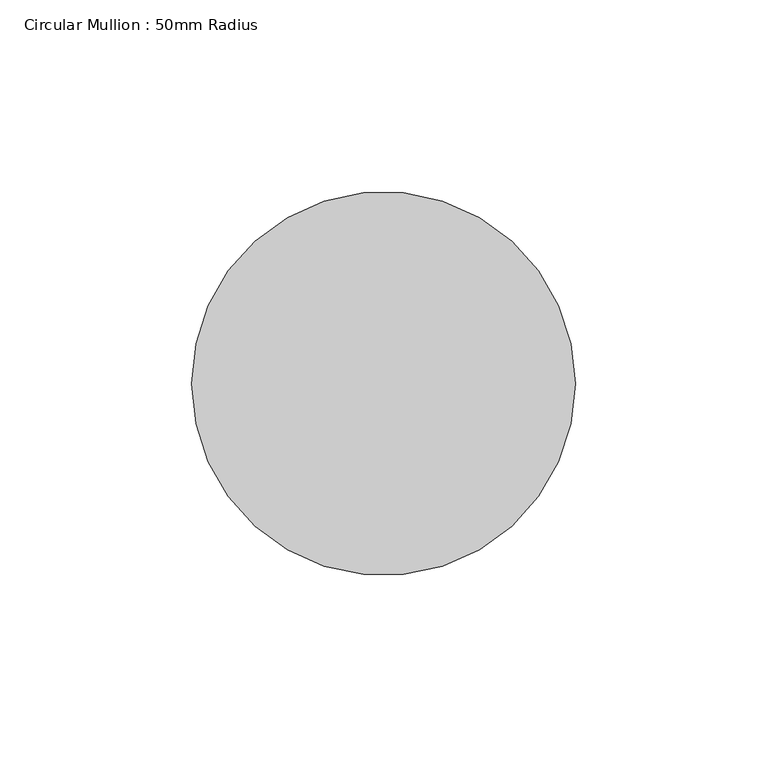
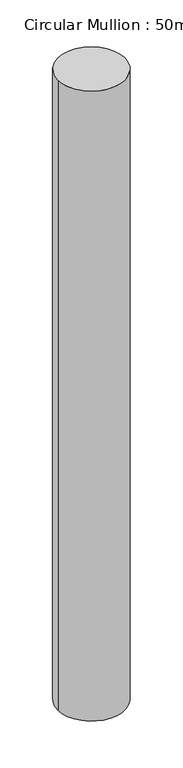
"""IFC4 building model written with IfcOpenShell, lengths in millimetres: member geometry, Circular Mullion : 50mm Radius."""

from ifc_helpers import new_model, si_unit, point, frame, origin, origin_2d, place, context, project, spatial, circle_curve, trimmed, segment, composite_curve, outline, extrude, source, transform, mapped, element, save


def circular_mullion_50mm_radius_3d0bf691(model_context):
    return source(origin(), model_context, "Body", "SweptSolid", [
        extrude(outline(composite_curve([segment(trimmed(circle_curve(origin_2d(), 50.0), [point((50.0, 0.0))], [point((-50.0, 0.0))], False, "CARTESIAN"), True, "CONTINUOUS"), segment(trimmed(circle_curve(origin_2d(), 50.0), [point((-50.0, 0.0))], [point((50.0, 0.0))], False, "CARTESIAN"), True, "CONTINUOUS")], self_intersect=False)), frame((0.0, 0.0, -993.8270485), z_axis=(0.0, 0.0, 1.0), x_axis=(1.0, 0.0, 0.0)), (0.0, 0.0, 1.0), 993.8270485),
    ])


if __name__ == "__main__":
    model = new_model("IFC4")
    model_context = context("Model", 3, world=origin())
    ifc_project = project(units=[si_unit("LENGTHUNIT", "METRE", prefix="MILLI")], contexts=[model_context])
    site = spatial("IfcSite", under=ifc_project)
    building = spatial("IfcBuilding", under=site)
    placement = place(None, origin())
    circular_mullion_50mm_radius_shape = circular_mullion_50mm_radius_3d0bf691(model_context)
    element("IfcMember", 1, ObjectType="Circular Mullion : 50mm Radius", at=placement, inside=building, context=model_context, shape_type="MappedRepresentation", body=[
        mapped(circular_mullion_50mm_radius_shape, transform((0.0, 0.0, 0.0), x_axis=(1.0, 0.0, 0.0), y_axis=(0.0, 1.0, 0.0), z_axis=(0.0, 0.0, 1.0))),
    ])
    save(model, "model.ifc")

# Revit data of these elements
# Type "Circular Mullion : 50mm Radius"
#   built-in parameter 1007350 = 0.164042 (stored number, unit not read)
# Element 1 (IfcMember, "Circular Mullion : 50mm Radius")
#   Materials on its faces: "Aluminium"
# Materials
#   "Aluminium": class "Metal", colour RGB 247 247 247, transparency 0, Description = "Aluminium 6061", Cost = 0
